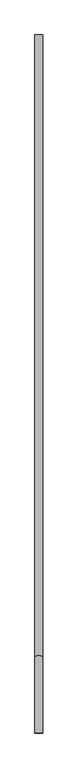
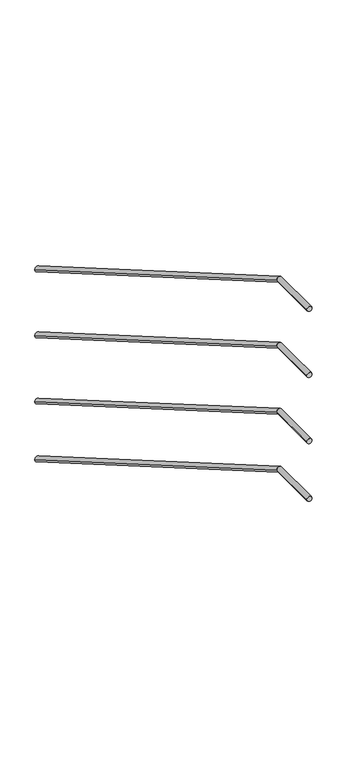
"""IFC4 building model written with IfcOpenShell, lengths in millimetres: railing geometry."""

from ifc_helpers import new_model, si_unit, frame, origin, place, context, project, spatial, circle_curve, ellipse_curve, source, transform, mapped, element, save
from ifc_brep_helpers import plane_surface, cylinder_surface, advanced_brep


def railing_778d8cd7(model_context):
    return source(origin(), model_context, "Body", "AdvancedBrep", [
        advanced_brep(
        [(-340.4, 15799.5208589, 5689.6773196), (-310.4, 15799.5208589, 5689.6773196), (-340.4, 13395.4833005, 7084.9618634), (-310.4, 13395.4833005, 7084.9618634), (-340.4, 13099.5208589, 7084.9618634), (-310.4, 13099.5208589, 7084.9618634)],
        [
            (0, 1, ellipse_curve(frame((-325.4, 15799.5208589, 5689.6773196), z_axis=(0.0, 1.0, 0.0), x_axis=(0.0, 0.0, -1.0)), 17.3433672, 15.0)),
            (1, 0, ellipse_curve(frame((-325.4, 15799.5208589, 5689.6773196), z_axis=(0.0, 1.0, 0.0), x_axis=(0.0, 0.0, -1.0)), 17.3433672, 15.0)),
            (0, 2),
            (2, 3, ellipse_curve(frame((-325.4, 13395.4833005, 7084.9618634), z_axis=(0.0, 0.9656303515230847, -0.2599192648062161), x_axis=(0.0, -0.2599192648062165, -0.9656303515230846)), 15.5338945, 15.0)),
            (3, 1),
            (3, 2, ellipse_curve(frame((-325.4, 13395.4833005, 7084.9618634), z_axis=(0.0, 0.9656303515230847, -0.2599192648062161), x_axis=(0.0, -0.2599192648062165, -0.9656303515230846)), 15.5338945, 15.0)),
            (4, 5, circle_curve(frame((-325.4, 13099.5208589, 7084.9618634), z_axis=(0.0, -1.0, 0.0), x_axis=(1.0, 0.0, 0.0)), 15.0)),
            (5, 4, circle_curve(frame((-325.4, 13099.5208589, 7084.9618634), z_axis=(0.0, -1.0, 0.0), x_axis=(1.0, 0.0, 0.0)), 15.0)),
            (2, 4),
            (5, 3),
        ],
        [
            plane_surface(frame((-325.4, 15799.5208589, 5707.0206869), z_axis=(0.0, 1.0, 0.0), x_axis=(0.0, 0.0, -1.0))),
            cylinder_surface(frame((-325.4, 15791.991281, 5694.0474276), z_axis=(0.0, 0.8648839515651924, -0.5019718620848963), x_axis=(1.0, 0.0, 0.0)), 15.0),
            plane_surface(frame((-325.4, 13099.5208589, 7099.9618634), z_axis=(0.0, -1.0, 0.0), x_axis=(0.0, 0.0, -1.0))),
            cylinder_surface(frame((-325.4, 13399.5208589, 7084.9618634), z_axis=(0.0, 1.0, 0.0), x_axis=(1.0, 0.0, 0.0)), 15.0),
        ],
        [
            (0, [[1, 2]]),
            (1, [[-1, 3, 4, 5]]),
            (1, [[-2, -5, 6, -3]]),
            (2, [[7, 8]]),
            (3, [[-4, 9, -8, 10]]),
            (3, [[-6, -10, -7, -9]]),
        ],
    ),
        advanced_brep(
        [(-340.4, 15799.5208589, 4889.6773196), (-310.4, 15799.5208589, 4889.6773196), (-340.4, 13395.4833005, 6284.9618634), (-310.4, 13395.4833005, 6284.9618634), (-340.4, 13099.5208589, 6284.9618634), (-310.4, 13099.5208589, 6284.9618634)],
        [
            (0, 1, ellipse_curve(frame((-325.4, 15799.5208589, 4889.6773196), z_axis=(0.0, 1.0, 0.0), x_axis=(0.0, 0.0, -1.0)), 17.3433672, 15.0)),
            (1, 0, ellipse_curve(frame((-325.4, 15799.5208589, 4889.6773196), z_axis=(0.0, 1.0, 0.0), x_axis=(0.0, 0.0, -1.0)), 17.3433672, 15.0)),
            (0, 2),
            (2, 3, ellipse_curve(frame((-325.4, 13395.4833005, 6284.9618634), z_axis=(0.0, 0.9656303515230847, -0.2599192648062161), x_axis=(0.0, -0.2599192648062165, -0.9656303515230846)), 15.5338945, 15.0)),
            (3, 1),
            (3, 2, ellipse_curve(frame((-325.4, 13395.4833005, 6284.9618634), z_axis=(0.0, 0.9656303515230847, -0.2599192648062161), x_axis=(0.0, -0.2599192648062165, -0.9656303515230846)), 15.5338945, 15.0)),
            (4, 5, circle_curve(frame((-325.4, 13099.5208589, 6284.9618634), z_axis=(0.0, -1.0, 0.0), x_axis=(1.0, 0.0, 0.0)), 15.0)),
            (5, 4, circle_curve(frame((-325.4, 13099.5208589, 6284.9618634), z_axis=(0.0, -1.0, 0.0), x_axis=(1.0, 0.0, 0.0)), 15.0)),
            (2, 4),
            (5, 3),
        ],
        [
            plane_surface(frame((-325.4, 15799.5208589, 4907.0206869), z_axis=(0.0, 1.0, 0.0), x_axis=(0.0, 0.0, -1.0))),
            cylinder_surface(frame((-325.4, 15791.991281, 4894.0474276), z_axis=(0.0, 0.8648839515651924, -0.5019718620848963), x_axis=(1.0, 0.0, 0.0)), 15.0),
            plane_surface(frame((-325.4, 13099.5208589, 6299.9618634), z_axis=(0.0, -1.0, 0.0), x_axis=(0.0, 0.0, -1.0))),
            cylinder_surface(frame((-325.4, 13399.5208589, 6284.9618634), z_axis=(0.0, 1.0, 0.0), x_axis=(1.0, 0.0, 0.0)), 15.0),
        ],
        [
            (0, [[1, 2]]),
            (1, [[-1, 3, 4, 5]]),
            (1, [[-2, -5, 6, -3]]),
            (2, [[7, 8]]),
            (3, [[-4, 9, -8, 10]]),
            (3, [[-6, -10, -7, -9]]),
        ],
    ),
        advanced_brep(
        [(-340.4, 15799.5208589, 5289.6773196), (-310.4, 15799.5208589, 5289.6773196), (-340.4, 13395.4833005, 6684.9618634), (-310.4, 13395.4833005, 6684.9618634), (-340.4, 13099.5208589, 6684.9618634), (-310.4, 13099.5208589, 6684.9618634)],
        [
            (0, 1, ellipse_curve(frame((-325.4, 15799.5208589, 5289.6773196), z_axis=(0.0, 1.0, 0.0), x_axis=(0.0, 0.0, -1.0)), 17.3433672, 15.0)),
            (1, 0, ellipse_curve(frame((-325.4, 15799.5208589, 5289.6773196), z_axis=(0.0, 1.0, 0.0), x_axis=(0.0, 0.0, -1.0)), 17.3433672, 15.0)),
            (0, 2),
            (2, 3, ellipse_curve(frame((-325.4, 13395.4833005, 6684.9618634), z_axis=(0.0, 0.9656303515230847, -0.2599192648062161), x_axis=(0.0, -0.2599192648062165, -0.9656303515230846)), 15.5338945, 15.0)),
            (3, 1),
            (3, 2, ellipse_curve(frame((-325.4, 13395.4833005, 6684.9618634), z_axis=(0.0, 0.9656303515230847, -0.2599192648062161), x_axis=(0.0, -0.2599192648062165, -0.9656303515230846)), 15.5338945, 15.0)),
            (4, 5, circle_curve(frame((-325.4, 13099.5208589, 6684.9618634), z_axis=(0.0, -1.0, 0.0), x_axis=(1.0, 0.0, 0.0)), 15.0)),
            (5, 4, circle_curve(frame((-325.4, 13099.5208589, 6684.9618634), z_axis=(0.0, -1.0, 0.0), x_axis=(1.0, 0.0, 0.0)), 15.0)),
            (2, 4),
            (5, 3),
        ],
        [
            plane_surface(frame((-325.4, 15799.5208589, 5307.0206869), z_axis=(0.0, 1.0, 0.0), x_axis=(0.0, 0.0, -1.0))),
            cylinder_surface(frame((-325.4, 15791.991281, 5294.0474276), z_axis=(0.0, 0.8648839515651924, -0.5019718620848963), x_axis=(1.0, 0.0, 0.0)), 15.0),
            plane_surface(frame((-325.4, 13099.5208589, 6699.9618634), z_axis=(0.0, -1.0, 0.0), x_axis=(0.0, 0.0, -1.0))),
            cylinder_surface(frame((-325.4, 13399.5208589, 6684.9618634), z_axis=(0.0, 1.0, 0.0), x_axis=(1.0, 0.0, 0.0)), 15.0),
        ],
        [
            (0, [[1, 2]]),
            (1, [[-1, 3, 4, 5]]),
            (1, [[-2, -5, 6, -3]]),
            (2, [[7, 8]]),
            (3, [[-4, 9, -8, 10]]),
            (3, [[-6, -10, -7, -9]]),
        ],
    ),
        advanced_brep(
        [(-340.4, 15799.5208589, 4539.6773196), (-310.4, 15799.5208589, 4539.6773196), (-340.4, 13395.4833005, 5934.9618634), (-310.4, 13395.4833005, 5934.9618634), (-340.4, 13099.5208589, 5934.9618634), (-310.4, 13099.5208589, 5934.9618634)],
        [
            (0, 1, ellipse_curve(frame((-325.4, 15799.5208589, 4539.6773196), z_axis=(0.0, 1.0, 0.0), x_axis=(0.0, 0.0, -1.0)), 17.3433672, 15.0)),
            (1, 0, ellipse_curve(frame((-325.4, 15799.5208589, 4539.6773196), z_axis=(0.0, 1.0, 0.0), x_axis=(0.0, 0.0, -1.0)), 17.3433672, 15.0)),
            (0, 2),
            (2, 3, ellipse_curve(frame((-325.4, 13395.4833005, 5934.9618634), z_axis=(0.0, 0.9656303515230847, -0.2599192648062161), x_axis=(0.0, -0.2599192648062165, -0.9656303515230846)), 15.5338945, 15.0)),
            (3, 1),
            (3, 2, ellipse_curve(frame((-325.4, 13395.4833005, 5934.9618634), z_axis=(0.0, 0.9656303515230847, -0.2599192648062161), x_axis=(0.0, -0.2599192648062165, -0.9656303515230846)), 15.5338945, 15.0)),
            (4, 5, circle_curve(frame((-325.4, 13099.5208589, 5934.9618634), z_axis=(0.0, -1.0, 0.0), x_axis=(1.0, 0.0, 0.0)), 15.0)),
            (5, 4, circle_curve(frame((-325.4, 13099.5208589, 5934.9618634), z_axis=(0.0, -1.0, 0.0), x_axis=(1.0, 0.0, 0.0)), 15.0)),
            (2, 4),
            (5, 3),
        ],
        [
            plane_surface(frame((-325.4, 15799.5208589, 4557.0206869), z_axis=(0.0, 1.0, 0.0), x_axis=(0.0, 0.0, -1.0))),
            cylinder_surface(frame((-325.4, 15791.991281, 4544.0474276), z_axis=(0.0, 0.8648839515651924, -0.5019718620848963), x_axis=(1.0, 0.0, 0.0)), 15.0),
            plane_surface(frame((-325.4, 13099.5208589, 5949.9618634), z_axis=(0.0, -1.0, 0.0), x_axis=(0.0, 0.0, -1.0))),
            cylinder_surface(frame((-325.4, 13399.5208589, 5934.9618634), z_axis=(0.0, 1.0, 0.0), x_axis=(1.0, 0.0, 0.0)), 15.0),
        ],
        [
            (0, [[1, 2]]),
            (1, [[-1, 3, 4, 5]]),
            (1, [[-2, -5, 6, -3]]),
            (2, [[7, 8]]),
            (3, [[-4, 9, -8, 10]]),
            (3, [[-6, -10, -7, -9]]),
        ],
    ),
    ])


if __name__ == "__main__":
    model = new_model("IFC4")
    model_context = context("Model", 3, world=origin())
    ifc_project = project(units=[si_unit("LENGTHUNIT", "METRE", prefix="MILLI")], contexts=[model_context])
    site = spatial("IfcSite", under=ifc_project)
    building = spatial("IfcBuilding", under=site)
    placement = place(None, origin())
    railing_shape = railing_778d8cd7(model_context)
    element("IfcRailing", 1, at=placement, inside=building, context=model_context, shape_type="MappedRepresentation", body=[
        mapped(railing_shape, transform((0.0, 0.0, 0.0), x_axis=(1.0, 0.0, 0.0), y_axis=(0.0, 1.0, 0.0), z_axis=(0.0, 0.0, 1.0))),
    ])
    save(model, "model.ifc")
